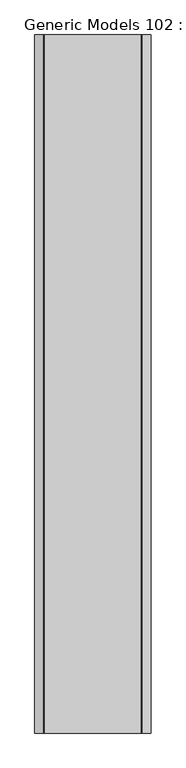
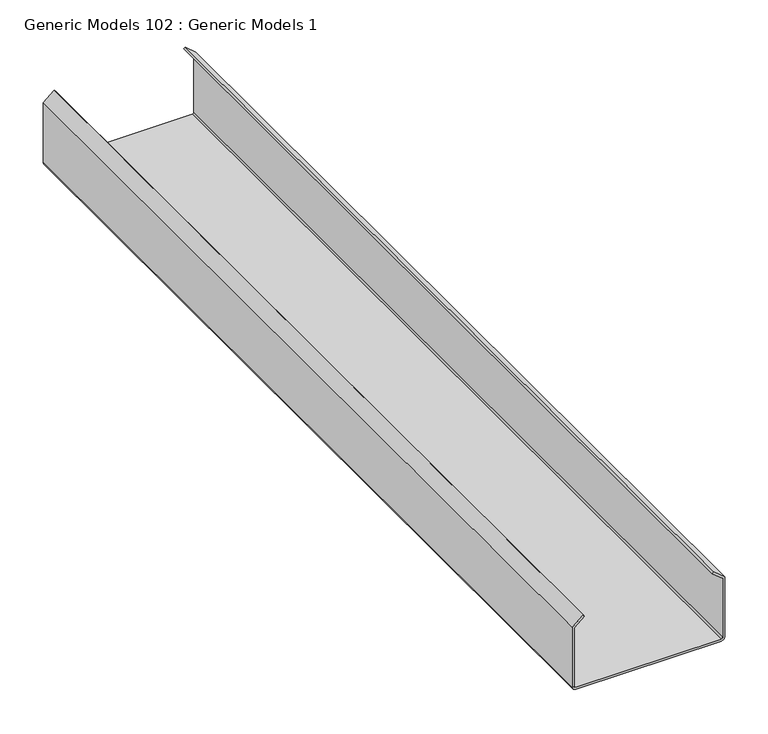
"""IFC4 building model written with IfcOpenShell, lengths in millimetres: proxy geometry, Generic Models 102 : Generic Models 1."""

from ifc_helpers import new_model, si_unit, point, frame, frame_2d, origin, place, context, project, spatial, polyline, circle_curve, trimmed, segment, composite_curve, outline, extrude, source, transform, mapped, element, save


def generic_models_102_generic_models_1_8a2dd616(model_context):
    return source(origin(), model_context, "Body", "SweptSolid", [
        extrude(outline(composite_curve([segment(polyline([(4498.578125, 52222.4), (4510.823229, 52207.8068534), (4508.6950617, 52206.021109), (4497.282664, 52219.621875), (4414.3677682, 52219.621875)]), True, "CONTINUOUS"), segment(trimmed(circle_curve(frame_2d((4414.4412941, 52217.6381931)), 1.9850441), [point((4414.3677682, 52219.621875))], [point((4412.45625, 52217.6381931))], True, "CARTESIAN"), True, "CONTINUOUS"), segment(polyline([(4412.45625, 52217.6381931), (4412.45625, 52023.9610661)]), True, "CONTINUOUS"), segment(trimmed(circle_curve(frame_2d((4414.4419899, 52023.9610661)), 1.9857399), [point((4412.45625, 52023.9610661))], [point((4414.3365981, 52021.978125))], True, "CARTESIAN"), True, "CONTINUOUS"), segment(polyline([(4414.3365981, 52021.978125), (4497.282664, 52021.978125), (4508.718285, 52035.6065673), (4510.8464522, 52033.820823), (4498.578125, 52019.2), (4414.440625, 52019.2)]), True, "CONTINUOUS"), segment(trimmed(circle_curve(frame_2d((4414.440625, 52023.9625)), 4.7625), [point((4414.440625, 52019.2))], [point((4409.678125, 52023.9625))], False, "CARTESIAN"), True, "CONTINUOUS"), segment(polyline([(4409.678125, 52023.9625), (4409.678125, 52217.6375)]), True, "CONTINUOUS"), segment(trimmed(circle_curve(frame_2d((4414.440625, 52217.6375)), 4.7625), [point((4409.678125, 52217.6375))], [point((4414.440625, 52222.4))], False, "CARTESIAN"), True, "CONTINUOUS"), segment(polyline([(4414.440625, 52222.4), (4498.578125, 52222.4)]), True, "CONTINUOUS")], self_intersect=False)), frame((0.0, 0.0, 0.0), z_axis=(0.0, 1.0, 0.0), x_axis=(0.0, 0.0, 1.0)), (0.0, 0.0, 1.0), 1219.2),
    ])


if __name__ == "__main__":
    model = new_model("IFC4")
    model_context = context("Model", 3, world=origin())
    ifc_project = project(units=[si_unit("LENGTHUNIT", "METRE", prefix="MILLI")], contexts=[model_context])
    site = spatial("IfcSite", under=ifc_project)
    building = spatial("IfcBuilding", under=site)
    placement = place(None, origin())
    generic_models_102_generic_models_1_shape = generic_models_102_generic_models_1_8a2dd616(model_context)
    element("IfcBuildingElementProxy", 1, Name="Generic Models 102 : Generic Models 1", ObjectType="Generic Models 102 : Generic Models 1", at=placement, inside=building, context=model_context, shape_type="MappedRepresentation", body=[
        mapped(generic_models_102_generic_models_1_shape, transform((0.0, 0.0, 0.0), x_axis=(1.0, 0.0, 0.0), y_axis=(0.0, 1.0, 0.0), z_axis=(0.0, 0.0, 1.0))),
    ])
    save(model, "model.ifc")

# Revit data of these elements
# Element 1 (IfcBuildingElementProxy, "Generic Models 102 : Generic Models 1")
#   Materials on its faces: "EXISTING GIRT"
# Materials
#   "EXISTING GIRT": class "Metal", colour RGB 87 87 87, transparency 0, Description = "Carbon steel", Cost = 0
